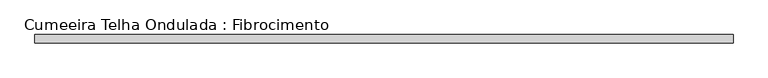
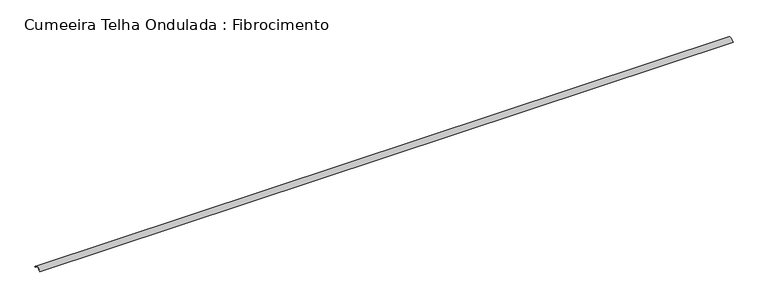
"""IFC4 building model written with IfcOpenShell, lengths in millimetres: beam geometry, Cumeeira Telha Ondulada : Fibrocimento."""

from ifc_helpers import new_model, si_unit, point, frame, frame_2d, origin, place, context, project, spatial, polyline, circle_curve, trimmed, segment, composite_curve, outline, extrude, source, transform, mapped, element, save


def cumeeira_telha_ondulada_fibrocimento_c9eafb3e(model_context):
    return source(origin(), model_context, "Body", "SweptSolid", [
        extrude(outline(composite_curve([segment(polyline([(58.3970135, 42.4437972), (53.9055884, 40.2467307)]), True, "CONTINUOUS"), segment(trimmed(circle_curve(frame_2d((-1.6029865, 13.0936483)), 61.7939461), [point((53.9055884, 40.2467307))], [point((-57.1115615, 40.2467307))], True, "CARTESIAN"), True, "CONTINUOUS"), segment(polyline([(-57.1115615, 40.2467307), (-61.6029865, 42.4437972)]), True, "CONTINUOUS"), segment(trimmed(circle_curve(frame_2d((-1.6029865, 13.0936483)), 66.7939461), [point((-61.6029865, 42.4437972))], [point((58.3970135, 42.4437972))], False, "CARTESIAN"), True, "CONTINUOUS")], self_intersect=False)), frame((-4969.5, 0.0, 0.0), z_axis=(1.0, 0.0, 0.0), x_axis=(0.0, 1.0, 0.0)), (0.0, 0.0, 1.0), 9939.0),
    ])


if __name__ == "__main__":
    model = new_model("IFC4")
    model_context = context("Model", 3, world=origin())
    ifc_project = project(units=[si_unit("LENGTHUNIT", "METRE", prefix="MILLI")], contexts=[model_context])
    site = spatial("IfcSite", under=ifc_project)
    building = spatial("IfcBuilding", under=site)
    placement = place(None, origin())
    cumeeira_telha_ondulada_fibrocimento_shape = cumeeira_telha_ondulada_fibrocimento_c9eafb3e(model_context)
    element("IfcBeam", 1, ObjectType="Cumeeira Telha Ondulada : Fibrocimento", at=placement, inside=building, context=model_context, shape_type="MappedRepresentation", body=[
        mapped(cumeeira_telha_ondulada_fibrocimento_shape, transform((0.0, 0.0, 0.0), x_axis=(1.0, 0.0, 0.0), y_axis=(0.0, 1.0, 0.0), z_axis=(0.0, 0.0, 1.0))),
    ])
    save(model, "model.ifc")

# Revit data of these elements
# Type "Cumeeira Telha Ondulada : Fibrocimento"
#   Cost = 5
#   Length [instance default] = 1.524 m
#   b = 0.07 m
#   h = 0.16 m
#   Structural Material = .TELHA DE FIBROCIMENTO
#   Assembly Code = ""
# Element 1 (IfcBeam, "Cumeeira Telha Ondulada : Fibrocimento")
#   Materials on its faces: ".TELHA DE FIBROCIMENTO"
# Materials
#   ".TELHA DE FIBROCIMENTO": class "CC_TELHADO", colour RGB 77 77 76, transparency 0, Description = "TELHA ONDULADA FIBROCIMENTO", Cost = 0
